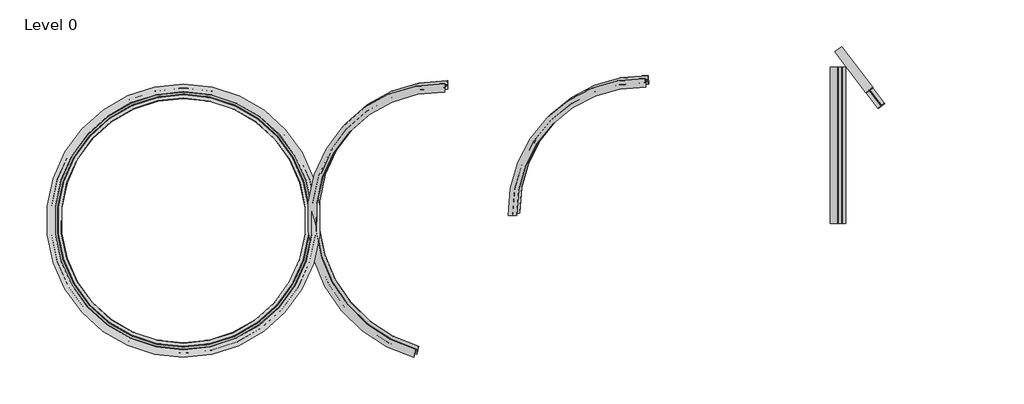
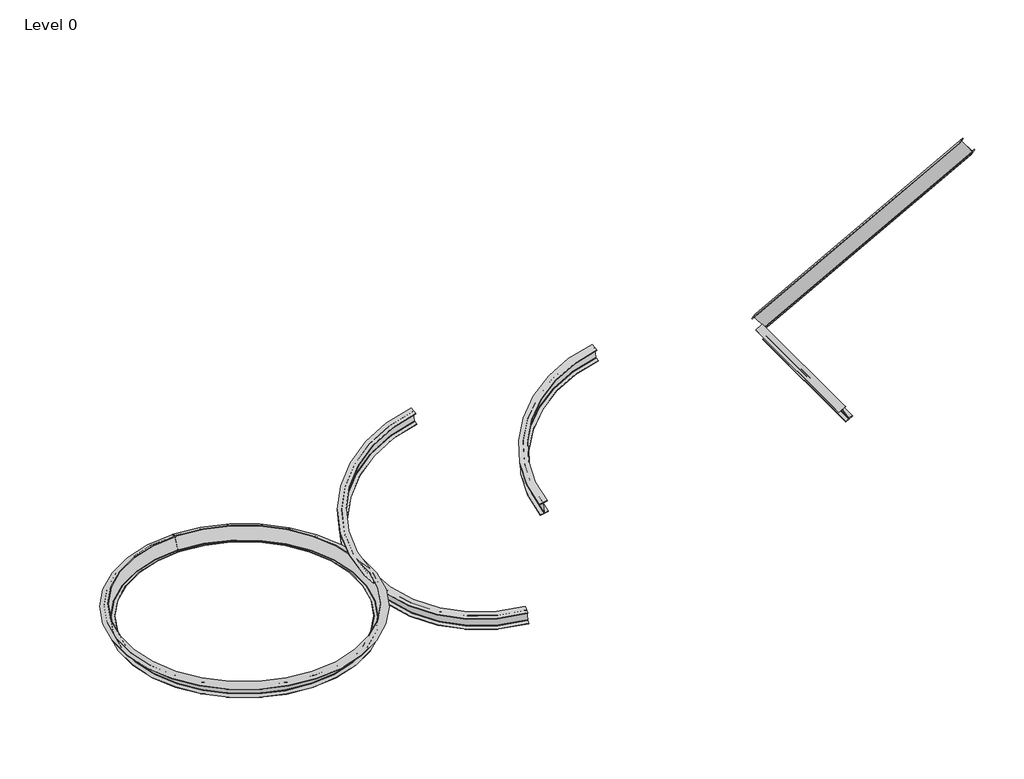
# One storey: 5 beams.
"""IFC4 building model written with IfcOpenShell, lengths in millimetres."""

import ifcopenshell
import ifcopenshell.guid

model = None  # the IFC model being written
_history = None  # IfcOwnerHistory: only IFC2X3 demands one
_inside = {}  # id of a spatial element -> (the spatial element, [elements in it])
_under = {}  # id of a project, library or spatial element -> (it, [spatial elements below it])
_declared = {}  # id of a project -> (the project, [libraries it declares])
_typed = {}  # id of a type object -> (the type object, [elements of that type])
_made_of = {}  # id of a material, layer set ... -> (it, [elements and type objects made of it])


def new_model(schema):
    """Start an empty IFC model of exactly this schema.

    Asked for "IFC4X3", IfcOpenShell would pick the latest addendum, in which some entities
    have other attributes; the version numbers below select the first issue.
    IFC2X3 requires an IfcOwnerHistory on every rooted entity: one is made here for all.
    """
    global model, _history
    if schema == "IFC4X3":
        model = ifcopenshell.file(schema_version=(4, 3, 0, 0))
    else:
        model = ifcopenshell.file(schema=schema)
    _inside.clear()
    _under.clear()
    _declared.clear()
    _typed.clear()
    _made_of.clear()
    _history = None
    if model.schema == "IFC2X3":
        org = make("IfcOrganization", Name="unknown")
        user = make(
            "IfcPersonAndOrganization",
            ThePerson=make("IfcPerson", FamilyName="unknown"),
            TheOrganization=org,
        )
        app = make(
            "IfcApplication",
            ApplicationDeveloper=org,
            Version="unknown",
            ApplicationFullName="unknown",
            ApplicationIdentifier="unknown",
        )
        _history = make(
            "IfcOwnerHistory",
            OwningUser=user,
            OwningApplication=app,
            ChangeAction="ADDED",
            CreationDate=0,
        )
    return model


def make(cls, **values):
    """One entity of the class cls with the attributes given. An attribute that is None is left unset."""
    return model.create_entity(
        cls, **{name: value for name, value in values.items() if value is not None}
    )


def rooted(cls, **values):
    """An entity with a GlobalId (a new one), such as an element, a storey or a relation."""
    return make(cls, GlobalId=ifcopenshell.guid.new(), OwnerHistory=_history, **values)


def si_unit(unit_type, name, prefix=None):
    """IfcSIUnit, for example si_unit("LENGTHUNIT", "METRE", prefix="MILLI")."""
    return make("IfcSIUnit", UnitType=unit_type, Prefix=prefix, Name=name)


def assignment(units):
    """IfcUnitAssignment: the units of a project."""
    return None if units is None else make("IfcUnitAssignment", Units=units)


def point(xyz):
    """IfcCartesianPoint."""
    return None if xyz is None else make("IfcCartesianPoint", Coordinates=xyz)


def direction(xyz):
    """IfcDirection."""
    return None if xyz is None else make("IfcDirection", DirectionRatios=xyz)


def frame(location, z_axis=None, x_axis=None):
    """IfcAxis2Placement3D, a coordinate frame: its origin and axes. An axis left out is left unset."""
    return make(
        "IfcAxis2Placement3D",
        Location=point(location),
        Axis=direction(z_axis),
        RefDirection=direction(x_axis),
    )


def frame_2d(location, x_axis=None):
    """IfcAxis2Placement2D, a coordinate frame in the plane: its origin and x axis."""
    return make(
        "IfcAxis2Placement2D", Location=point(location), RefDirection=direction(x_axis)
    )


def origin():
    """The frame at (0, 0, 0) with its axes left unset."""
    return frame((0.0, 0.0, 0.0))


def place(relative_to, where):
    """IfcLocalPlacement: puts the frame where relative to a parent placement (None: the world)."""
    return make(
        "IfcLocalPlacement", PlacementRelTo=relative_to, RelativePlacement=where
    )


def context(
    kind, dimensions, precision=None, world=None, true_north=None, identifier=None
):
    """IfcGeometricRepresentationContext, for example the 3D "Model" context."""
    return make(
        "IfcGeometricRepresentationContext",
        ContextIdentifier=identifier,
        ContextType=kind,
        CoordinateSpaceDimension=dimensions,
        Precision=precision,
        WorldCoordinateSystem=world,
        TrueNorth=true_north,
    )


def project(units=None, contexts=None):
    """IfcProject with its units and contexts."""
    return rooted(
        "IfcProject",
        Name="project",
        RepresentationContexts=contexts,
        UnitsInContext=assignment(units),
    )


def spatial(cls, under=None, at=None, **own):
    """A site, building, storey or space (cls), placed at a placement, below another one or the project."""
    s = rooted(cls, ObjectPlacement=at, **own)
    if under is not None:
        _under.setdefault(under.id(), (under, []))[1].append(s)
    return s


def polyline(points):
    """IfcPolyline through the points."""
    return make("IfcPolyline", Points=[point(p) for p in points])


def circle_curve(where, radius):
    """IfcCircle in the frame where."""
    return make("IfcCircle", Position=where, Radius=radius)


def ellipse_curve(where, semi_axis1, semi_axis2):
    """IfcEllipse in the frame where."""
    return make(
        "IfcEllipse", Position=where, SemiAxis1=semi_axis1, SemiAxis2=semi_axis2
    )


def trimmed(basis, trim1, trim2, sense, master):
    """IfcTrimmedCurve: the piece of a basis curve between two trims."""
    return make(
        "IfcTrimmedCurve",
        BasisCurve=basis,
        Trim1=trim1,
        Trim2=trim2,
        SenseAgreement=sense,
        MasterRepresentation=master,
    )


def segment(curve, same_sense, transition):
    """IfcCompositeCurveSegment."""
    return make(
        "IfcCompositeCurveSegment",
        Transition=transition,
        SameSense=same_sense,
        ParentCurve=curve,
    )


def composite_curve(segments, self_intersect=None):
    """IfcCompositeCurve: segments joined end to end."""
    return make("IfcCompositeCurve", Segments=segments, SelfIntersect=self_intersect)


def outline(outer, holes=None, kind="AREA"):
    """IfcArbitraryClosedProfileDef: a profile drawn as a closed curve; with holes, ...WithVoids."""
    if holes is None:
        return make("IfcArbitraryClosedProfileDef", ProfileType=kind, OuterCurve=outer)
    return make(
        "IfcArbitraryProfileDefWithVoids",
        ProfileType=kind,
        OuterCurve=outer,
        InnerCurves=holes,
    )


def extrude(swept, where, along, depth):
    """IfcExtrudedAreaSolid: the profile swept, set in the frame where, extruded along a direction by depth."""
    return make(
        "IfcExtrudedAreaSolid",
        SweptArea=swept,
        Position=where,
        ExtrudedDirection=direction(along),
        Depth=depth,
    )


def shape(context_of_items, identifier, shape_type, items):
    """IfcShapeRepresentation: the items that make up one representation, for example the "Body"."""
    return make(
        "IfcShapeRepresentation",
        ContextOfItems=context_of_items,
        RepresentationIdentifier=identifier,
        RepresentationType=shape_type,
        Items=items,
    )


def source(mapping_origin, context_of_items, identifier, shape_type, items):
    """IfcRepresentationMap: a shape defined once, which mapped items show again and again."""
    return make(
        "IfcRepresentationMap",
        MappingOrigin=mapping_origin,
        MappedRepresentation=shape(context_of_items, identifier, shape_type, items),
    )


def transform(
    local_origin,
    x_axis=None,
    y_axis=None,
    z_axis=None,
    scale=None,
    scale2=None,
    scale3=None,
    uniform=True,
):
    """IfcCartesianTransformationOperator3D, or its non-uniform kind. x_axis, y_axis, z_axis: its Axis1, 2, 3."""
    if uniform:
        return make(
            "IfcCartesianTransformationOperator3D",
            Axis1=direction(x_axis),
            Axis2=direction(y_axis),
            LocalOrigin=point(local_origin),
            Scale=scale,
            Axis3=direction(z_axis),
        )
    return make(
        "IfcCartesianTransformationOperator3DnonUniform",
        Axis1=direction(x_axis),
        Axis2=direction(y_axis),
        LocalOrigin=point(local_origin),
        Scale=scale,
        Axis3=direction(z_axis),
        Scale2=scale2,
        Scale3=scale3,
    )


def mapped(mapping_source, mapping_target):
    """IfcMappedItem: shows the shape of a source again, moved by a transform."""
    return make(
        "IfcMappedItem", MappingSource=mapping_source, MappingTarget=mapping_target
    )


def made_of(thing, what):
    """Note that an element or type object is made of a material, layer set ...; save() writes the relation."""
    if what is not None:
        _made_of.setdefault(what.id(), (what, []))[1].append(thing)
    return thing


def element(
    cls,
    number,
    at=None,
    inside=None,
    cuts=None,
    type_object=None,
    material=None,
    context=None,
    identifier="Body",
    shape_type=None,
    held_by="IfcProductDefinitionShape",
    body=None,
    shapes=None,
    **own,
):
    """One element of the class cls, such as IfcWall. Its Tag is "e" and its number.

    at: its placement. inside: the storey or other place that contains it. cuts: it is an
    opening in that element (IfcRelVoidsElement). A single representation is given by context,
    identifier, shape_type and body (its items); several are given by shapes. held_by: the class
    of the entity that holds the representations. save() writes the other relations.
    """
    e = rooted(cls, Tag="e%d" % number, ObjectPlacement=at, **own)
    if body is not None:
        shapes = [shape(context, identifier, shape_type, body)]
    if shapes is not None:
        e.Representation = make(held_by, Representations=shapes)
    if inside is not None:
        _inside.setdefault(inside.id(), (inside, []))[1].append(e)
    if cuts is not None:
        rooted(
            "IfcRelVoidsElement", RelatingBuildingElement=cuts, RelatedOpeningElement=e
        )
    if type_object is not None:
        _typed.setdefault(type_object.id(), (type_object, []))[1].append(e)
    return made_of(e, material)


def aggregate(whole, parts):
    """IfcRelAggregates: a whole, such as a stair, and the parts it consists of."""
    return rooted("IfcRelAggregates", RelatingObject=whole, RelatedObjects=parts)


def save(model, path):
    """Write the relations noted so far, then the file.

    IfcRelAggregates (storeys below a building ...), IfcRelContainedInSpatialStructure (elements
    in a storey), IfcRelDefinesByType, IfcRelAssociatesMaterial and IfcRelDeclares: one each for
    every whole, place, type object, material and project.
    """
    for whole, parts in _under.values():
        aggregate(whole, parts)
    for where, things in _inside.values():
        rooted(
            "IfcRelContainedInSpatialStructure",
            RelatedElements=things,
            RelatingStructure=where,
        )
    for kind, things in _typed.values():
        rooted("IfcRelDefinesByType", RelatedObjects=things, RelatingType=kind)
    for what, things in _made_of.values():
        rooted("IfcRelAssociatesMaterial", RelatedObjects=things, RelatingMaterial=what)
    for by, libraries in _declared.values():
        rooted("IfcRelDeclares", RelatingContext=by, RelatedDefinitions=libraries)
    model.write(path)


def plane_surface(at):
    """IfcPlane: the flat surface through the origin of the frame at, square to its z axis."""
    return make("IfcPlane", Position=at)


def cylinder_surface(at, radius):
    """IfcCylindricalSurface: all points at the distance radius from the z axis of the frame at."""
    return make("IfcCylindricalSurface", Position=at, Radius=radius)


def revolved_surface(curve, axis_point, axis_direction):
    """IfcSurfaceOfRevolution: the curve turned about the line through axis_point along axis_direction."""
    return make(
        "IfcSurfaceOfRevolution",
        SweptCurve=make("IfcArbitraryOpenProfileDef", ProfileType="CURVE", Curve=curve),
        AxisPosition=make("IfcAxis1Placement", Location=point(axis_point), Axis=direction(axis_direction)),
    )


def advanced_brep(points, edges, surfaces, faces):
    """IfcAdvancedBrep: a solid bounded by faces that lie on surfaces and meet in shared edges.

    An edge is (start, end): straight between two places in points (the first is 0);
    or (start, end, curve); or (start, end, curve, False) where it runs against its curve.
    A face is (place in surfaces, loops), or (place, loops, False) where it looks against
    its surface's normal. A loop lists edges by number (the first is 1), with a minus sign
    where the edge is run from its end to its start. The first loop is the outer one.
    """
    corners = [point(p) for p in points]
    vertices = [make("IfcVertexPoint", VertexGeometry=c) for c in corners]
    made = []
    for start, end, *more in edges:
        made.append(
            make(
                "IfcEdgeCurve",
                EdgeStart=vertices[start],
                EdgeEnd=vertices[end],
                EdgeGeometry=more[0] if more else make("IfcPolyline", Points=[corners[start], corners[end]]),
                SameSense=more[1] if len(more) > 1 else True,
            )
        )
    hull = []
    for where, loops, *sense in faces:
        bounds = []
        for j, loop in enumerate(loops):
            ring = [make("IfcOrientedEdge", EdgeElement=made[abs(k) - 1], Orientation=k > 0) for k in loop]
            bounds.append(
                make(
                    "IfcFaceOuterBound" if j == 0 else "IfcFaceBound",
                    Bound=make("IfcEdgeLoop", EdgeList=ring),
                    Orientation=True,
                )
            )
        hull.append(make("IfcAdvancedFace", Bounds=bounds, FaceSurface=surfaces[where], SameSense=sense[0] if sense else True))
    return make("IfcAdvancedBrep", Outer=make("IfcClosedShell", CfsFaces=hull))


def ub_universal_beams_ub305x165x40_8b2c45c1(model_context):
    return source(origin(), model_context, "Body", "SweptSolid", [
        extrude(outline(composite_curve([segment(polyline([(82.5, -141.5), (82.5, -151.7), (-82.5, -151.7), (-82.5, -141.5), (-11.9, -141.5)]), True, "CONTINUOUS"), segment(trimmed(circle_curve(frame_2d((-11.9, -132.6)), 8.9), [point((-11.9, -141.5))], [point((-3.0, -132.6))], True, "CARTESIAN"), True, "CONTINUOUS"), segment(polyline([(-3.0, -132.6), (-3.0, 132.6)]), True, "CONTINUOUS"), segment(trimmed(circle_curve(frame_2d((-11.9, 132.6)), 8.9), [point((-3.0, 132.6))], [point((-11.9, 141.5))], True, "CARTESIAN"), True, "CONTINUOUS"), segment(polyline([(-11.9, 141.5), (-82.5, 141.5), (-82.5, 151.7), (82.5, 151.7), (82.5, 141.5), (11.9, 141.5)]), True, "CONTINUOUS"), segment(trimmed(circle_curve(frame_2d((11.9, 132.6)), 8.9), [point((11.9, 141.5))], [point((3.0, 132.6))], True, "CARTESIAN"), True, "CONTINUOUS"), segment(polyline([(3.0, 132.6), (3.0, -132.6)]), True, "CONTINUOUS"), segment(trimmed(circle_curve(frame_2d((11.9, -132.6)), 8.9), [point((3.0, -132.6))], [point((11.9, -141.5))], True, "CARTESIAN"), True, "CONTINUOUS"), segment(polyline([(11.9, -141.5), (82.5, -141.5)]), True, "CONTINUOUS")], self_intersect=False)), frame((-1500.0, 0.0, 0.0), z_axis=(1.0, 0.0, 0.0), x_axis=(0.0, 1.0, 0.0)), (0.0, 0.0, 1.0), 3000.0),
    ])


def ub_universal_beams_ub305x165x40_614cc3fe(model_context):
    return source(origin(), model_context, "Body", "SweptSolid", [
        extrude(outline(composite_curve([segment(polyline([(82.5, -141.5), (82.5, -151.7), (-82.5, -151.7), (-82.5, -141.5), (-11.9, -141.5)]), True, "CONTINUOUS"), segment(trimmed(circle_curve(frame_2d((-11.9, -132.6)), 8.9), [point((-11.9, -141.5))], [point((-3.0, -132.6))], True, "CARTESIAN"), True, "CONTINUOUS"), segment(polyline([(-3.0, -132.6), (-3.0, 132.6)]), True, "CONTINUOUS"), segment(trimmed(circle_curve(frame_2d((-11.9, 132.6)), 8.9), [point((-3.0, 132.6))], [point((-11.9, 141.5))], True, "CARTESIAN"), True, "CONTINUOUS"), segment(polyline([(-11.9, 141.5), (-82.5, 141.5), (-82.5, 151.7), (82.5, 151.7), (82.5, 141.5), (11.9, 141.5)]), True, "CONTINUOUS"), segment(trimmed(circle_curve(frame_2d((11.9, 132.6)), 8.9), [point((11.9, 141.5))], [point((3.0, 132.6))], True, "CARTESIAN"), True, "CONTINUOUS"), segment(polyline([(3.0, 132.6), (3.0, -132.6)]), True, "CONTINUOUS"), segment(trimmed(circle_curve(frame_2d((11.9, -132.6)), 8.9), [point((3.0, -132.6))], [point((11.9, -141.5))], True, "CARTESIAN"), True, "CONTINUOUS"), segment(polyline([(11.9, -141.5), (82.5, -141.5)]), True, "CONTINUOUS")], self_intersect=False)), frame((-3226.45, 0.0, 0.0), z_axis=(1.0, 0.0, 0.0), x_axis=(0.0, 1.0, 0.0)), (0.0, 0.0, 1.0), 6452.9),
    ])


def ub_universal_beams_ub305x165x40_b211cafa(model_context):
    return source(origin(), model_context, "Body", "AdvancedBrep", [
        advanced_brep(
        [(-9.2813175, 14.9526552, -163.1085585), (-9.0434318, -49.0322323, -133.2717092), (-9.0274272, -53.3370394, -121.4442673), (-9.444114, 58.7405491, 118.9085578), (-9.4880863, 70.5679092, 123.2133946), (-9.725972, 134.5527967, 93.3765453), (-9.7419984, 138.8634732, 102.6208847), (-9.1860332, -10.6762782, 172.3528979), (-9.1700068, -14.9869547, 163.1085585), (-9.4078925, 48.9979329, 133.2717092), (-9.4238971, 53.3027399, 121.4442673), (-9.0072103, -58.7748485, -118.9085578), (-8.9632381, -70.6022086, -123.2133946), (-8.7253523, -134.5870962, -93.3765453), (-8.7093259, -138.8977726, -102.6208847), (-9.2652911, 10.6419787, -172.3528979), (0.0, 14.9699084, -163.1085585), (0.0, 10.6592021, -172.3528979), (0.0, -138.8815827, -102.6208847), (0.0, -134.5708765, -93.3765453), (0.0, -70.5855467, -123.2133946), (0.0, -58.7581049, -118.9085578), (0.0, 53.3202581, 121.4442673), (0.0, 49.0154214, 133.2717092), (0.0, -14.9699084, 163.1085585), (0.0, -10.6592021, 172.3528979), (0.0, 138.8815827, 102.6208847), (0.0, 134.5708765, 93.3765453), (0.0, 70.5855467, 123.2133946), (0.0, 58.7581049, 118.9085578), (0.0, -53.3202581, -121.4442673), (0.0, -49.0154214, -133.2717092)],
        [
            (0, 1),
            (1, 2, circle_curve(frame((-9.0574157, -45.2709558, -125.2055699), z_axis=(-0.9999930888962334, -0.0037178165326446095, 0.0), x_axis=(0.0033694860743094072, -0.9063015234494892, 0.4226182617406991)), 8.9)),
            (2, 3),
            (3, 4, circle_curve(frame((-9.4741024, 66.8066326, 115.1472552), z_axis=(-0.9999930888962334, -0.0037178165326453875, 0.0), x_axis=(0.003369486074310112, -0.9063015234494892, 0.42261826174069916)), 8.9)),
            (4, 5),
            (5, 6),
            (6, 7),
            (7, 8),
            (8, 9),
            (9, 10, circle_curve(frame((-9.3939087, 45.2366564, 125.2055699), z_axis=(-0.9999930888962334, -0.0037178165326453875, 0.0), x_axis=(0.003369486074310112, -0.9063015234494892, 0.42261826174069916)), 8.9)),
            (10, 11),
            (11, 12, circle_curve(frame((-8.9772219, -66.8409321, -115.1472552), z_axis=(-0.9999930888962334, -0.0037178165326446095, 0.0), x_axis=(0.0033694860743094072, -0.9063015234494892, 0.4226182617406991)), 8.9)),
            (12, 13),
            (13, 14),
            (14, 15),
            (15, 0),
            (16, 17),
            (17, 18),
            (18, 19),
            (19, 20),
            (20, 21, circle_curve(frame((0.0, -66.8242442, -115.1472552), z_axis=(1.0000000000000002, 0.0, 0.0), x_axis=(0.0, -0.9063077870366502, 0.4226182617406991)), 8.9)),
            (21, 22),
            (22, 23, circle_curve(frame((0.0, 45.2541188, 125.2055699), z_axis=(1.0000000000000002, 0.0, 0.0), x_axis=(0.0, -0.9063077870366502, 0.42261826174069916)), 8.9)),
            (23, 24),
            (24, 25),
            (25, 26),
            (26, 27),
            (27, 28),
            (28, 29, circle_curve(frame((0.0, 66.8242442, 115.1472552), z_axis=(1.0000000000000002, 0.0, 0.0), x_axis=(0.0, -0.9063077870366502, 0.42261826174069916)), 8.9)),
            (29, 30),
            (30, 31, circle_curve(frame((0.0, -45.2541188, -125.2055699), z_axis=(1.0000000000000002, 0.0, 0.0), x_axis=(0.0, -0.9063077870366502, 0.4226182617406991)), 8.9)),
            (31, 16),
            (0, 16, circle_curve(frame((0.0, -2481.473222, -163.1085585), z_axis=(0.0, 0.0, 1.0), x_axis=(-0.9999930888962332, -0.0037178165326318038, 0.0)), 2496.4431304)),
            (31, 1, circle_curve(frame((0.0, -2481.473222, -133.2717092), z_axis=(0.0, 0.0, -1.0), x_axis=(-0.9999930888962332, -0.0037178165326318038, 0.0)), 2432.4578006)),
            (30, 2, circle_curve(frame((0.0, -2481.473222, -121.4442673), z_axis=(0.0, 0.0, -1.0), x_axis=(-0.9999930888962332, -0.0037178165326318038, 0.0)), 2428.1529638)),
            (29, 3, circle_curve(frame((0.0, -2481.473222, 118.9085578), z_axis=(0.0, 0.0, -1.0), x_axis=(-0.9999930888962332, -0.0037178165326318038, 0.0)), 2540.2313268)),
            (28, 4, circle_curve(frame((0.0, -2481.473222, 123.2133946), z_axis=(0.0, 0.0, -1.0), x_axis=(-0.9999930888962332, -0.0037178165326318038, 0.0)), 2552.0587687)),
            (27, 5, circle_curve(frame((0.0, -2481.473222, 93.3765453), z_axis=(0.0, 0.0, -1.0), x_axis=(-0.9999930888962332, -0.0037178165326318038, 0.0)), 2616.0440984)),
            (26, 6, circle_curve(frame((0.0, -2481.473222, 102.6208847), z_axis=(0.0, 0.0, -1.0), x_axis=(-0.9999930888962332, -0.0037178165326318038, 0.0)), 2620.3548047)),
            (25, 7, circle_curve(frame((0.0, -2481.473222, 172.3528979), z_axis=(0.0, 0.0, -1.0), x_axis=(-0.9999930888962332, -0.0037178165326318038, 0.0)), 2470.8140198)),
            (24, 8, circle_curve(frame((0.0, -2481.473222, 163.1085585), z_axis=(0.0, 0.0, -1.0), x_axis=(-0.9999930888962332, -0.0037178165326318038, 0.0)), 2466.5033136)),
            (23, 9, circle_curve(frame((0.0, -2481.473222, 133.2717092), z_axis=(0.0, 0.0, -1.0), x_axis=(-0.9999930888962332, -0.0037178165326318038, 0.0)), 2530.4886433)),
            (22, 10, circle_curve(frame((0.0, -2481.473222, 121.4442673), z_axis=(0.0, 0.0, -1.0), x_axis=(-0.9999930888962332, -0.0037178165326318038, 0.0)), 2534.7934801)),
            (21, 11, circle_curve(frame((0.0, -2481.473222, -118.9085578), z_axis=(0.0, 0.0, -1.0), x_axis=(-0.9999930888962332, -0.0037178165326318038, 0.0)), 2422.7151171)),
            (20, 12, circle_curve(frame((0.0, -2481.473222, -123.2133946), z_axis=(0.0, 0.0, -1.0), x_axis=(-0.9999930888962332, -0.0037178165326318038, 0.0)), 2410.8876753)),
            (19, 13, circle_curve(frame((0.0, -2481.473222, -93.3765453), z_axis=(0.0, 0.0, -1.0), x_axis=(-0.9999930888962332, -0.0037178165326318038, 0.0)), 2346.9023455)),
            (18, 14, circle_curve(frame((0.0, -2481.473222, -102.6208847), z_axis=(0.0, 0.0, -1.0), x_axis=(-0.9999930888962332, -0.0037178165326318038, 0.0)), 2342.5916392)),
            (17, 15, circle_curve(frame((0.0, -2481.473222, -172.3528979), z_axis=(0.0, 0.0, -1.0), x_axis=(-0.9999930888962332, -0.0037178165326318038, 0.0)), 2492.1324241)),
        ],
        [
            plane_surface(frame((-9.2256622, -0.0171497, 0.0), z_axis=(0.9999930888962332, 0.0037178165326321104, 0.0), x_axis=(-0.0015712171604918153, 0.42261534098203835, 0.9063077870366502))),
            plane_surface(frame((0.0, 0.0, 0.0), z_axis=(-1.0, 0.0, 0.0), x_axis=(0.0, 0.422618261740699, 0.9063077870366502))),
            revolved_surface(polyline([(-2432.4409896, -2490.5166538, -133.2717092), (-2496.4258772, -2490.7545395, -163.1085585)]), (0.0, -2481.473222, 0.0), (0.0, 0.0, -1.0)),
            revolved_surface(trimmed(ellipse_curve(frame((-2436.2022662, -2490.5306376, -125.2055699), z_axis=(-0.0037178165326371983, 0.9999930888962334, 0.0), x_axis=(0.9063015234494892, 0.00336948607430269, 0.4226182617406992)), 8.9, 8.9), [point((-2428.1361826, -2490.5006492, -121.4442673))], [point((-2432.4409896, -2490.5166538, -133.2717092))], True, "CARTESIAN"), (0.0, -2481.473222, 0.0), (0.0, 0.0, -1.0)),
            revolved_surface(polyline([(-2540.213771, -2490.917336, 118.9085578), (-2428.1361826, -2490.5006492, -121.4442673)]), (0.0, -2481.473222, 0.0), (0.0, 0.0, -1.0)),
            revolved_surface(trimmed(ellipse_curve(frame((-2548.2798546, -2490.9473244, 115.1472552), z_axis=(-0.003717816532637976, 0.9999930888962334, 0.0), x_axis=(0.9063015234494892, 0.0033694860743033947, 0.4226182617406993)), 8.9, 8.9), [point((-2552.0411311, -2490.9613082, 123.2133946))], [point((-2540.213771, -2490.917336, 118.9085578))], True, "CARTESIAN"), (0.0, -2481.473222, 0.0), (0.0, 0.0, -1.0)),
            revolved_surface(polyline([(-2616.0260187, -2491.199194, 93.3765453), (-2552.0411311, -2490.9613082, 123.2133946)]), (0.0, -2481.473222, 0.0), (0.0, 0.0, -1.0)),
            revolved_surface(polyline([(-2620.3366952, -2491.2152204, 102.6208847), (-2616.0260187, -2491.199194, 93.3765453)]), (0.0, -2481.473222, 0.0), (0.0, 0.0, -1.0)),
            revolved_surface(polyline([(-2470.7969438, -2490.6592552, 172.3528979), (-2620.3366952, -2491.2152204, 102.6208847)]), (0.0, -2481.473222, 0.0), (0.0, 0.0, -1.0)),
            revolved_surface(polyline([(-2466.4862673, -2490.6432288, 163.1085585), (-2470.7969438, -2490.6592552, 172.3528979)]), (0.0, -2481.473222, 0.0), (0.0, 0.0, -1.0)),
            revolved_surface(polyline([(-2530.4711549, -2490.8811145, 133.2717092), (-2466.4862673, -2490.6432288, 163.1085585)]), (0.0, -2481.473222, 0.0), (0.0, 0.0, -1.0)),
            revolved_surface(trimmed(ellipse_curve(frame((-2526.7098783, -2490.8671306, 125.2055699), z_axis=(-0.003717816532637976, 0.9999930888962334, 0.0), x_axis=(0.9063015234494892, 0.0033694860743033947, 0.4226182617406993)), 8.9, 8.9), [point((-2534.7759619, -2490.8971191, 121.4442673))], [point((-2530.4711549, -2490.8811145, 133.2717092))], True, "CARTESIAN"), (0.0, -2481.473222, 0.0), (0.0, 0.0, -1.0)),
            revolved_surface(polyline([(-2422.6983735, -2490.4804323, -118.9085578), (-2534.7759619, -2490.8971191, 121.4442673)]), (0.0, -2481.473222, 0.0), (0.0, 0.0, -1.0)),
            revolved_surface(trimmed(ellipse_curve(frame((-2414.6322899, -2490.4504439, -115.1472552), z_axis=(-0.0037178165326371983, 0.9999930888962334, 0.0), x_axis=(0.9063015234494892, 0.00336948607430269, 0.4226182617406992)), 8.9, 8.9), [point((-2410.8710134, -2490.43646, -123.2133946))], [point((-2422.6983735, -2490.4804323, -118.9085578))], True, "CARTESIAN"), (0.0, -2481.473222, 0.0), (0.0, 0.0, -1.0)),
            revolved_surface(polyline([(-2346.8861258, -2490.1985743, -93.3765453), (-2410.8710134, -2490.43646, -123.2133946)]), (0.0, -2481.473222, 0.0), (0.0, 0.0, -1.0)),
            revolved_surface(polyline([(-2342.5754493, -2490.1825479, -102.6208847), (-2346.8861258, -2490.1985743, -93.3765453)]), (0.0, -2481.473222, 0.0), (0.0, 0.0, -1.0)),
            revolved_surface(polyline([(-2492.1152007, -2490.7385131, -172.3528979), (-2342.5754493, -2490.1825479, -102.6208847)]), (0.0, -2481.473222, 0.0), (0.0, 0.0, -1.0)),
            revolved_surface(polyline([(-2496.4258772, -2490.7545395, -163.1085585), (-2492.1152007, -2490.7385131, -172.3528979)]), (0.0, -2481.473222, 0.0), (0.0, 0.0, -1.0)),
        ],
        [
            (0, [[1, 2, 3, 4, 5, 6, 7, 8, 9, 10, 11, 12, 13, 14, 15, 16]]),
            (1, [[17, 18, 19, 20, 21, 22, 23, 24, 25, 26, 27, 28, 29, 30, 31, 32]]),
            (2, [[-1, 33, -32, 34]]),
            (3, [[-2, -34, -31, 35]]),
            (4, [[-3, -35, -30, 36]]),
            (5, [[-4, -36, -29, 37]]),
            (6, [[-5, -37, -28, 38]]),
            (7, [[-6, -38, -27, 39]]),
            (8, [[-7, -39, -26, 40]]),
            (9, [[-8, -40, -25, 41]]),
            (10, [[-9, -41, -24, 42]]),
            (11, [[-10, -42, -23, 43]]),
            (12, [[-11, -43, -22, 44]]),
            (13, [[-12, -44, -21, 45]]),
            (14, [[-13, -45, -20, 46]]),
            (15, [[-14, -46, -19, 47]]),
            (16, [[-15, -47, -18, 48]]),
            (17, [[-16, -48, -17, -33]]),
        ],
    ),
    ])


def ub_universal_beams_ub305x165x40_4e4f8f72(model_context):
    return source(origin(), model_context, "Body", "AdvancedBrep", [
        advanced_brep(
        [(2724.4689627, -2641.9689627, -141.5), (2653.8689627, -2641.9689627, -141.5), (2644.9689627, -2641.9689627, -132.6), (2644.9689627, -2641.9689627, 132.6), (2653.8689627, -2641.9689627, 141.5), (2724.4689627, -2641.9689627, 141.5), (2724.4689627, -2641.9689627, 151.7), (2559.4689627, -2641.9689627, 151.7), (2559.4689627, -2641.9689627, 141.5), (2630.0689627, -2641.9689627, 141.5), (2638.9689627, -2641.9689627, 132.6), (2638.9689627, -2641.9689627, -132.6), (2630.0689627, -2641.9689627, -141.5), (2559.4689627, -2641.9689627, -141.5), (2559.4689627, -2641.9689627, -151.7), (2724.4689627, -2641.9689627, -151.7), (-2633.0924312, -1942.2866222, -141.5), (-2633.0924312, -1942.2866222, -151.7), (-2473.6264005, -1984.6609666, -151.7), (-2473.6264005, -1984.6609666, -141.5), (-2541.8585324, -1966.5298835, -141.5), (-2550.4600335, -1964.244237, -132.6), (-2550.4600335, -1964.244237, 132.6), (-2541.8585324, -1966.5298835, 141.5), (-2473.6264005, -1984.6609666, 141.5), (-2473.6264005, -1984.6609666, 151.7), (-2633.0924312, -1942.2866222, 151.7), (-2633.0924312, -1942.2866222, 141.5), (-2564.8602993, -1960.4177053, 141.5), (-2556.2587982, -1962.7033518, 132.6), (-2556.2587982, -1962.7033518, -132.6), (-2564.8602993, -1960.4177053, -141.5)],
        [
            (0, 1),
            (1, 2, circle_curve(frame((2653.8689627, -2641.9689627, -132.6), z_axis=(0.0, 1.0, 0.0), x_axis=(-1.0, 0.0, 0.0)), 8.9)),
            (2, 3),
            (3, 4, circle_curve(frame((2653.8689627, -2641.9689627, 132.6), z_axis=(0.0, 1.0, 0.0), x_axis=(-1.0, 0.0, 0.0)), 8.9)),
            (4, 5),
            (5, 6),
            (6, 7),
            (7, 8),
            (8, 9),
            (9, 10, circle_curve(frame((2630.0689627, -2641.9689627, 132.6), z_axis=(0.0, 1.0, 0.0), x_axis=(-1.0, 0.0, 0.0)), 8.9)),
            (10, 11),
            (11, 12, circle_curve(frame((2630.0689627, -2641.9689627, -132.6), z_axis=(0.0, 1.0, 0.0), x_axis=(-1.0, 0.0, 0.0)), 8.9)),
            (12, 13),
            (13, 14),
            (14, 15),
            (15, 0),
            (16, 17),
            (17, 18),
            (18, 19),
            (19, 20),
            (20, 21, circle_curve(frame((-2541.8585324, -1966.5298835, -132.6), z_axis=(0.2568142086103926, 0.9664607918875021, 0.0), x_axis=(0.9664607918875021, -0.2568142086103926, 0.0)), 8.9)),
            (21, 22),
            (22, 23, circle_curve(frame((-2541.8585324, -1966.5298835, 132.6), z_axis=(0.2568142086103926, 0.9664607918875021, 0.0), x_axis=(0.9664607918875021, -0.2568142086103926, 0.0)), 8.9)),
            (23, 24),
            (24, 25),
            (25, 26),
            (26, 27),
            (27, 28),
            (28, 29, circle_curve(frame((-2564.8602993, -1960.4177053, 132.6), z_axis=(0.2568142086103926, 0.9664607918875021, 0.0), x_axis=(0.9664607918875021, -0.2568142086103926, 0.0)), 8.9)),
            (29, 30),
            (30, 31, circle_curve(frame((-2564.8602993, -1960.4177053, -132.6), z_axis=(0.2568142086103926, 0.9664607918875021, 0.0), x_axis=(0.9664607918875021, -0.2568142086103926, 0.0)), 8.9)),
            (31, 16),
            (0, 16, circle_curve(frame((0.0, -2641.9689627, -141.5), z_axis=(0.0, 0.0, 1.0), x_axis=(0.0, 1.0, 0.0)), 2724.4689627)),
            (31, 1, circle_curve(frame((0.0, -2641.9689627, -141.5), z_axis=(0.0, 0.0, -1.0), x_axis=(0.0, 1.0, 0.0)), 2653.8689627)),
            (30, 2, circle_curve(frame((0.0, -2641.9689627, -132.6), z_axis=(0.0, 0.0, -1.0), x_axis=(0.0, 1.0, 0.0)), 2644.9689627)),
            (29, 3, circle_curve(frame((0.0, -2641.9689627, 132.6), z_axis=(0.0, 0.0, -1.0), x_axis=(0.0, 1.0, 0.0)), 2644.9689627)),
            (28, 4, circle_curve(frame((0.0, -2641.9689627, 141.5), z_axis=(0.0, 0.0, -1.0), x_axis=(0.0, 1.0, 0.0)), 2653.8689627)),
            (27, 5, circle_curve(frame((0.0, -2641.9689627, 141.5), z_axis=(0.0, 0.0, -1.0), x_axis=(0.0, 1.0, 0.0)), 2724.4689627)),
            (26, 6, circle_curve(frame((0.0, -2641.9689627, 151.7), z_axis=(0.0, 0.0, -1.0), x_axis=(0.0, 1.0, 0.0)), 2724.4689627)),
            (25, 7, circle_curve(frame((0.0, -2641.9689627, 151.7), z_axis=(0.0, 0.0, -1.0), x_axis=(0.0, 1.0, 0.0)), 2559.4689627)),
            (24, 8, circle_curve(frame((0.0, -2641.9689627, 141.5), z_axis=(0.0, 0.0, -1.0), x_axis=(0.0, 1.0, 0.0)), 2559.4689627)),
            (23, 9, circle_curve(frame((0.0, -2641.9689627, 141.5), z_axis=(0.0, 0.0, -1.0), x_axis=(0.0, 1.0, 0.0)), 2630.0689627)),
            (22, 10, circle_curve(frame((0.0, -2641.9689627, 132.6), z_axis=(0.0, 0.0, -1.0), x_axis=(0.0, 1.0, 0.0)), 2638.9689627)),
            (21, 11, circle_curve(frame((0.0, -2641.9689627, -132.6), z_axis=(0.0, 0.0, -1.0), x_axis=(0.0, 1.0, 0.0)), 2638.9689627)),
            (20, 12, circle_curve(frame((0.0, -2641.9689627, -141.5), z_axis=(0.0, 0.0, -1.0), x_axis=(0.0, 1.0, 0.0)), 2630.0689627)),
            (19, 13, circle_curve(frame((0.0, -2641.9689627, -141.5), z_axis=(0.0, 0.0, -1.0), x_axis=(0.0, 1.0, 0.0)), 2559.4689627)),
            (18, 14, circle_curve(frame((0.0, -2641.9689627, -151.7), z_axis=(0.0, 0.0, -1.0), x_axis=(0.0, 1.0, 0.0)), 2559.4689627)),
            (17, 15, circle_curve(frame((0.0, -2641.9689627, -151.7), z_axis=(0.0, 0.0, -1.0), x_axis=(0.0, 1.0, 0.0)), 2724.4689627)),
        ],
        [
            plane_surface(frame((2641.9689627, -2641.9689627, 0.0), z_axis=(0.0, -1.0, 0.0), x_axis=(0.0, 0.0, 1.0))),
            plane_surface(frame((-2553.3594159, -1963.4737944, 0.0), z_axis=(-0.25681420861039306, -0.9664607918875021, 0.0), x_axis=(0.0, 0.0, 1.0))),
            plane_surface(frame((0.0, -2641.9689627, -141.5), z_axis=(0.0, 0.0, 1.0), x_axis=(0.0, 1.0, 0.0))),
            revolved_surface(trimmed(ellipse_curve(frame((0.0, 11.9, -132.6), z_axis=(1.0, 0.0, 0.0), x_axis=(0.0, -1.0, 0.0)), 8.9, 8.9), [point((0.0, 3.0, -132.6))], [point((0.0, 11.9, -141.5))], True, "CARTESIAN"), (0.0, -2641.9689627, 0.0), (0.0, 0.0, -1.0)),
            cylinder_surface(frame((0.0, -2641.9689627, 0.0), z_axis=(0.0, 0.0, -1.0), x_axis=(0.0, 1.0, 0.0)), 2644.9689627),
            revolved_surface(trimmed(ellipse_curve(frame((0.0, 11.9, 132.6), z_axis=(1.0, 0.0, 0.0), x_axis=(0.0, -1.0, 0.0)), 8.9, 8.9), [point((0.0, 11.9, 141.5))], [point((0.0, 3.0, 132.6))], True, "CARTESIAN"), (0.0, -2641.9689627, 0.0), (0.0, 0.0, -1.0)),
            plane_surface(frame((0.0, -2641.9689627, 141.5), z_axis=(0.0, 0.0, -1.0), x_axis=(0.0, 1.0, 0.0))),
            cylinder_surface(frame((0.0, -2641.9689627, 0.0), z_axis=(0.0, 0.0, -1.0), x_axis=(0.0, 1.0, 0.0)), 2724.4689627),
            plane_surface(frame((0.0, -2641.9689627, 151.7), z_axis=(0.0, 0.0, 1.0), x_axis=(0.0, 1.0, 0.0))),
            revolved_surface(polyline([(0.0, -82.5, 141.5), (0.0, -82.5, 151.7)]), (0.0, -2641.9689627, 0.0), (0.0, 0.0, -1.0)),
            revolved_surface(trimmed(ellipse_curve(frame((0.0, -11.9, 132.6), z_axis=(1.0, 0.0, 0.0), x_axis=(0.0, -1.0, 0.0)), 8.9, 8.9), [point((0.0, -3.0, 132.6))], [point((0.0, -11.9, 141.5))], True, "CARTESIAN"), (0.0, -2641.9689627, 0.0), (0.0, 0.0, -1.0)),
            revolved_surface(polyline([(0.0, -3.0, -132.6), (0.0, -3.0, 132.6)]), (0.0, -2641.9689627, 0.0), (0.0, 0.0, -1.0)),
            revolved_surface(trimmed(ellipse_curve(frame((0.0, -11.9, -132.6), z_axis=(1.0, 0.0, 0.0), x_axis=(0.0, -1.0, 0.0)), 8.9, 8.9), [point((0.0, -11.9, -141.5))], [point((0.0, -3.0, -132.6))], True, "CARTESIAN"), (0.0, -2641.9689627, 0.0), (0.0, 0.0, -1.0)),
            revolved_surface(polyline([(0.0, -82.5, -151.7), (0.0, -82.5, -141.5)]), (0.0, -2641.9689627, 0.0), (0.0, 0.0, -1.0)),
            plane_surface(frame((0.0, -2641.9689627, -151.7), z_axis=(0.0, 0.0, -1.0), x_axis=(0.0, 1.0, 0.0))),
        ],
        [
            (0, [[1, 2, 3, 4, 5, 6, 7, 8, 9, 10, 11, 12, 13, 14, 15, 16]]),
            (1, [[17, 18, 19, 20, 21, 22, 23, 24, 25, 26, 27, 28, 29, 30, 31, 32]]),
            (2, [[-1, 33, -32, 34]]),
            (3, [[-2, -34, -31, 35]]),
            (4, [[-3, -35, -30, 36]]),
            (5, [[-4, -36, -29, 37]]),
            (6, [[-5, -37, -28, 38]]),
            (7, [[-6, -38, -27, 39]]),
            (8, [[-7, -39, -26, 40]]),
            (9, [[-8, -40, -25, 41]]),
            (6, [[-9, -41, -24, 42]]),
            (10, [[-10, -42, -23, 43]]),
            (11, [[-11, -43, -22, 44]]),
            (12, [[-12, -44, -21, 45]]),
            (2, [[-13, -45, -20, 46]]),
            (13, [[-14, -46, -19, 47]]),
            (14, [[-15, -47, -18, 48]]),
            (7, [[-16, -48, -17, -33]]),
        ],
    ),
    ])


def ub_universal_beams_ub305x165x40_a7bc032b(model_context):
    return source(origin(), model_context, "Body", "AdvancedBrep", [
        advanced_brep(
        [(2724.4689627, -2641.9689627, -141.5), (2653.8689627, -2641.9689627, -141.5), (2644.9689627, -2641.9689627, -132.6), (2644.9689627, -2641.9689627, 132.6), (2653.8689627, -2641.9689627, 141.5), (2724.4689627, -2641.9689627, 141.5), (2724.4689627, -2641.9689627, 151.7), (2559.4689627, -2641.9689627, 151.7), (2559.4689627, -2641.9689627, 141.5), (2630.0689627, -2641.9689627, 141.5), (2638.9689627, -2641.9689627, 132.6), (2638.9689627, -2641.9689627, -132.6), (2630.0689627, -2641.9689627, -141.5), (2559.4689627, -2641.9689627, -141.5), (2559.4689627, -2641.9689627, -151.7), (2724.4689627, -2641.9689627, -151.7), (0.0, 82.5, -141.5), (0.0, 82.5, -151.7), (0.0, -82.5, -151.7), (0.0, -82.5, -141.5), (0.0, -11.9, -141.5), (0.0, -3.0, -132.6), (0.0, -3.0, 132.6), (0.0, -11.9, 141.5), (0.0, -82.5, 141.5), (0.0, -82.5, 151.7), (0.0, 82.5, 151.7), (0.0, 82.5, 141.5), (0.0, 11.9, 141.5), (0.0, 3.0, 132.6), (0.0, 3.0, -132.6), (0.0, 11.9, -141.5)],
        [
            (0, 1),
            (1, 2, circle_curve(frame((2653.8689627, -2641.9689627, -132.6), z_axis=(0.0, 1.0, 0.0), x_axis=(-1.0, 0.0, 0.0)), 8.9)),
            (2, 3),
            (3, 4, circle_curve(frame((2653.8689627, -2641.9689627, 132.6), z_axis=(0.0, 1.0, 0.0), x_axis=(-1.0, 0.0, 0.0)), 8.9)),
            (4, 5),
            (5, 6),
            (6, 7),
            (7, 8),
            (8, 9),
            (9, 10, circle_curve(frame((2630.0689627, -2641.9689627, 132.6), z_axis=(0.0, 1.0, 0.0), x_axis=(-1.0, 0.0, 0.0)), 8.9)),
            (10, 11),
            (11, 12, circle_curve(frame((2630.0689627, -2641.9689627, -132.6), z_axis=(0.0, 1.0, 0.0), x_axis=(-1.0, 0.0, 0.0)), 8.9)),
            (12, 13),
            (13, 14),
            (14, 15),
            (15, 0),
            (16, 17),
            (17, 18),
            (18, 19),
            (19, 20),
            (20, 21, circle_curve(frame((0.0, -11.9, -132.6), z_axis=(1.0, 0.0, 0.0), x_axis=(0.0, -1.0, 0.0)), 8.9)),
            (21, 22),
            (22, 23, circle_curve(frame((0.0, -11.9, 132.6), z_axis=(1.0, 0.0, 0.0), x_axis=(0.0, -1.0, 0.0)), 8.9)),
            (23, 24),
            (24, 25),
            (25, 26),
            (26, 27),
            (27, 28),
            (28, 29, circle_curve(frame((0.0, 11.9, 132.6), z_axis=(1.0, 0.0, 0.0), x_axis=(0.0, -1.0, 0.0)), 8.9)),
            (29, 30),
            (30, 31, circle_curve(frame((0.0, 11.9, -132.6), z_axis=(1.0, 0.0, 0.0), x_axis=(0.0, -1.0, 0.0)), 8.9)),
            (31, 16),
            (0, 16, circle_curve(frame((0.0, -2641.9689627, -141.5), z_axis=(0.0, 0.0, 1.0), x_axis=(0.0, 1.0, 0.0)), 2724.4689627)),
            (31, 1, circle_curve(frame((0.0, -2641.9689627, -141.5), z_axis=(0.0, 0.0, -1.0), x_axis=(0.0, 1.0, 0.0)), 2653.8689627)),
            (30, 2, circle_curve(frame((0.0, -2641.9689627, -132.6), z_axis=(0.0, 0.0, -1.0), x_axis=(0.0, 1.0, 0.0)), 2644.9689627)),
            (29, 3, circle_curve(frame((0.0, -2641.9689627, 132.6), z_axis=(0.0, 0.0, -1.0), x_axis=(0.0, 1.0, 0.0)), 2644.9689627)),
            (28, 4, circle_curve(frame((0.0, -2641.9689627, 141.5), z_axis=(0.0, 0.0, -1.0), x_axis=(0.0, 1.0, 0.0)), 2653.8689627)),
            (27, 5, circle_curve(frame((0.0, -2641.9689627, 141.5), z_axis=(0.0, 0.0, -1.0), x_axis=(0.0, 1.0, 0.0)), 2724.4689627)),
            (26, 6, circle_curve(frame((0.0, -2641.9689627, 151.7), z_axis=(0.0, 0.0, -1.0), x_axis=(0.0, 1.0, 0.0)), 2724.4689627)),
            (25, 7, circle_curve(frame((0.0, -2641.9689627, 151.7), z_axis=(0.0, 0.0, -1.0), x_axis=(0.0, 1.0, 0.0)), 2559.4689627)),
            (24, 8, circle_curve(frame((0.0, -2641.9689627, 141.5), z_axis=(0.0, 0.0, -1.0), x_axis=(0.0, 1.0, 0.0)), 2559.4689627)),
            (23, 9, circle_curve(frame((0.0, -2641.9689627, 141.5), z_axis=(0.0, 0.0, -1.0), x_axis=(0.0, 1.0, 0.0)), 2630.0689627)),
            (22, 10, circle_curve(frame((0.0, -2641.9689627, 132.6), z_axis=(0.0, 0.0, -1.0), x_axis=(0.0, 1.0, 0.0)), 2638.9689627)),
            (21, 11, circle_curve(frame((0.0, -2641.9689627, -132.6), z_axis=(0.0, 0.0, -1.0), x_axis=(0.0, 1.0, 0.0)), 2638.9689627)),
            (20, 12, circle_curve(frame((0.0, -2641.9689627, -141.5), z_axis=(0.0, 0.0, -1.0), x_axis=(0.0, 1.0, 0.0)), 2630.0689627)),
            (19, 13, circle_curve(frame((0.0, -2641.9689627, -141.5), z_axis=(0.0, 0.0, -1.0), x_axis=(0.0, 1.0, 0.0)), 2559.4689627)),
            (18, 14, circle_curve(frame((0.0, -2641.9689627, -151.7), z_axis=(0.0, 0.0, -1.0), x_axis=(0.0, 1.0, 0.0)), 2559.4689627)),
            (17, 15, circle_curve(frame((0.0, -2641.9689627, -151.7), z_axis=(0.0, 0.0, -1.0), x_axis=(0.0, 1.0, 0.0)), 2724.4689627)),
        ],
        [
            plane_surface(frame((2641.9689627, -2641.9689627, 0.0), z_axis=(0.0, -1.0, 0.0), x_axis=(0.0, 0.0, 1.0))),
            plane_surface(frame((0.0, 0.0, 0.0), z_axis=(-1.0, 0.0, 0.0), x_axis=(0.0, 0.0, 1.0))),
            plane_surface(frame((0.0, -2641.9689627, -141.5), z_axis=(0.0, 0.0, 1.0), x_axis=(0.0, 1.0, 0.0))),
            revolved_surface(trimmed(ellipse_curve(frame((0.0, 11.9, -132.6), z_axis=(1.0, 0.0, 0.0), x_axis=(0.0, -1.0, 0.0)), 8.9, 8.9), [point((0.0, 3.0, -132.6))], [point((0.0, 11.9, -141.5))], True, "CARTESIAN"), (0.0, -2641.9689627, 0.0), (0.0, 0.0, -1.0)),
            cylinder_surface(frame((0.0, -2641.9689627, 0.0), z_axis=(0.0, 0.0, -1.0), x_axis=(0.0, 1.0, 0.0)), 2644.9689627),
            revolved_surface(trimmed(ellipse_curve(frame((0.0, 11.9, 132.6), z_axis=(1.0, 0.0, 0.0), x_axis=(0.0, -1.0, 0.0)), 8.9, 8.9), [point((0.0, 11.9, 141.5))], [point((0.0, 3.0, 132.6))], True, "CARTESIAN"), (0.0, -2641.9689627, 0.0), (0.0, 0.0, -1.0)),
            plane_surface(frame((0.0, -2641.9689627, 141.5), z_axis=(0.0, 0.0, -1.0), x_axis=(0.0, 1.0, 0.0))),
            cylinder_surface(frame((0.0, -2641.9689627, 0.0), z_axis=(0.0, 0.0, -1.0), x_axis=(0.0, 1.0, 0.0)), 2724.4689627),
            plane_surface(frame((0.0, -2641.9689627, 151.7), z_axis=(0.0, 0.0, 1.0), x_axis=(0.0, 1.0, 0.0))),
            revolved_surface(polyline([(0.0, -82.5, 141.5), (0.0, -82.5, 151.7)]), (0.0, -2641.9689627, 0.0), (0.0, 0.0, -1.0)),
            revolved_surface(trimmed(ellipse_curve(frame((0.0, -11.9, 132.6), z_axis=(1.0, 0.0, 0.0), x_axis=(0.0, -1.0, 0.0)), 8.9, 8.9), [point((0.0, -3.0, 132.6))], [point((0.0, -11.9, 141.5))], True, "CARTESIAN"), (0.0, -2641.9689627, 0.0), (0.0, 0.0, -1.0)),
            revolved_surface(polyline([(0.0, -3.0, -132.6), (0.0, -3.0, 132.6)]), (0.0, -2641.9689627, 0.0), (0.0, 0.0, -1.0)),
            revolved_surface(trimmed(ellipse_curve(frame((0.0, -11.9, -132.6), z_axis=(1.0, 0.0, 0.0), x_axis=(0.0, -1.0, 0.0)), 8.9, 8.9), [point((0.0, -11.9, -141.5))], [point((0.0, -3.0, -132.6))], True, "CARTESIAN"), (0.0, -2641.9689627, 0.0), (0.0, 0.0, -1.0)),
            revolved_surface(polyline([(0.0, -82.5, -151.7), (0.0, -82.5, -141.5)]), (0.0, -2641.9689627, 0.0), (0.0, 0.0, -1.0)),
            plane_surface(frame((0.0, -2641.9689627, -151.7), z_axis=(0.0, 0.0, -1.0), x_axis=(0.0, 1.0, 0.0))),
        ],
        [
            (0, [[1, 2, 3, 4, 5, 6, 7, 8, 9, 10, 11, 12, 13, 14, 15, 16]]),
            (1, [[17, 18, 19, 20, 21, 22, 23, 24, 25, 26, 27, 28, 29, 30, 31, 32]]),
            (2, [[-1, 33, -32, 34]]),
            (3, [[-2, -34, -31, 35]]),
            (4, [[-3, -35, -30, 36]]),
            (5, [[-4, -36, -29, 37]]),
            (6, [[-5, -37, -28, 38]]),
            (7, [[-6, -38, -27, 39]]),
            (8, [[-7, -39, -26, 40]]),
            (9, [[-8, -40, -25, 41]]),
            (6, [[-9, -41, -24, 42]]),
            (10, [[-10, -42, -23, 43]]),
            (11, [[-11, -43, -22, 44]]),
            (12, [[-12, -44, -21, 45]]),
            (2, [[-13, -45, -20, 46]]),
            (13, [[-14, -46, -19, 47]]),
            (14, [[-15, -47, -18, 48]]),
            (7, [[-16, -48, -17, -33]]),
        ],
    ),
    ])


model = new_model("IFC4")

# Units and contexts
model_context = context("Model", 3, world=origin())
ifc_project = project(units=[si_unit("LENGTHUNIT", "METRE", prefix="MILLI")], contexts=[model_context])

# Site, building, storey
site = spatial("IfcSite", under=ifc_project)
building = spatial("IfcBuilding", under=site)
storey = spatial("IfcBuildingStorey", under=building, Name="Level 0", Elevation=0.0)

# Beams
placement = place(None, origin())
ub_universal_beams_ub305x165x40_shape = ub_universal_beams_ub305x165x40_8b2c45c1(model_context)
element("IfcBeam", 1, ObjectType="UB-Universal Beams : UB305x165x40", at=placement, inside=storey, context=model_context, shape_type="MappedRepresentation", body=[
    mapped(ub_universal_beams_ub305x165x40_shape, transform((-14924.15, 5000.0, -131.3760538), x_axis=(0.0, 1.0, 0.0), y_axis=(-0.8660254037844388, 0.0, -0.49999999999999956), z_axis=(-0.49999999999999956, 0.0, 0.8660254037844388))),
])
ub_universal_beams_ub305x165x40_2_shape = ub_universal_beams_ub305x165x40_614cc3fe(model_context)
element("IfcBeam", 2, ObjectType="UB-Universal Beams : UB305x165x40", at=placement, inside=storey, context=model_context, shape_type="MappedRepresentation", body=[
    mapped(ub_universal_beams_ub305x165x40_2_shape, transform((-13620.5487861, 5121.1664701, 2404.1025892), x_axis=(-0.38043838153140086, 0.5048587841568978, -0.7748446592171796), y_axis=(-0.7986355100472944, -0.6018150231520465, 0.0), z_axis=(-0.46631315652602645, 0.6188184596213342, 0.632151685976248))),
])
ub_universal_beams_ub305x165x40_3_shape = ub_universal_beams_ub305x165x40_b211cafa(model_context)
element("IfcBeam", 3, ObjectType="UB-Universal Beams : UB305x165x40", at=placement, inside=storey, context=model_context, shape_type="MappedRepresentation", body=[
    mapped(ub_universal_beams_ub305x165x40_3_shape, transform((-27445.1899256, 6037.6373109, -137.4868913), x_axis=(0.9999930888962332, -0.003717816532617128, 0.0), y_axis=(0.003717816532617128, 0.9999930888962332, 0.0), z_axis=(0.0, 0.0, 1.0))),
])
ub_universal_beams_ub305x165x40_4_shape = ub_universal_beams_ub305x165x40_4e4f8f72(model_context)
element("IfcBeam", 4, ObjectType="UB-Universal Beams : UB305x165x40", at=placement, inside=storey, context=model_context, shape_type="MappedRepresentation", body=[
    mapped(ub_universal_beams_ub305x165x40_4_shape, transform((-24971.2903516, 3584.890887, -146.1656669), x_axis=(-0.018241045185027685, 0.9817589548149711, 0.18925279102611284), y_axis=(-0.9817589548149698, 0.018241045185031876, -0.18925279102612044), z_axis=(-0.18925279102612083, -0.18925279102611245, 0.9635179096299407))),
])
ub_universal_beams_ub305x165x40_5_shape = ub_universal_beams_ub305x165x40_a7bc032b(model_context)
element("IfcBeam", 5, ObjectType="UB-Universal Beams : UB305x165x40", at=placement, inside=storey, context=model_context, shape_type="MappedRepresentation", body=[
    mapped(ub_universal_beams_ub305x165x40_5_shape, transform((-21128.4413369, 3680.9711055, -146.1656669), x_axis=(-0.01824104518504623, 0.9817589548149572, 0.18925279102618278), y_axis=(-0.981758954814956, 0.018241045185040994, -0.1892527910261913), z_axis=(-0.18925279102619078, -0.1892527910261833, 0.963517909629913))),
])

save(model, "model.ifc")

# Revit data of these elements
# Project information
#   Project Issue Date = "Issue Date"
#   Project Status = "Project Status"
#   Client Name = "Owner"
#   Project Address = "Enter address here"
#   Project Name = "Project Name"
#   Project Number = "0001"
# Type "UB-Universal Beams : UB305x165x40"
#   Section Name Key = "UB305X165X40"
#   Width = 16.5 cm
#   Web Thickness = 0.6 cm
#   Web Fillet = 0.89 cm
#   Warping Constant = 164000.0 cm⁶
#   Torsional Moment of Inertia = 14.70 cm⁴
#   Section Area = 51.3 cm²
#   Plastic Modulus weak axis = 142.0 cm³
#   Plastic Modulus strong axis = 623.0 cm³
#   Nominal Weight = 40.2999 kgf/m
#   Moment of Inertia weak axis = 764.00 cm⁴
#   Moment of Inertia strong axis = 8503.00 cm⁴
#   Height = 30.34 cm
#   Flange Thickness = 1.02 cm
#   Elastic Modulus weak axis = 92.6 cm³
#   Elastic Modulus strong axis = 560.0 cm³
#   Centroid Vertical = 15.17 cm
#   Centroid Horizontal = 8.25 cm
#   Bolt Spacing = 9.0 cm
#   Length [instance default] = 1500 mm
#   Structural Material [instance default] = Metal - Steel 43-275
#   Type Comments = ""
#   Assembly Code = ""
# Element 1 (IfcBeam, "UB-Universal Beams : UB305x165x40")
#   SpeckleObjectUpdateDescription = "change cross section angle"
#   SpeckleObjectTestNumber = 4
#   Structural Material = Metal - Steel 43-275
#   Phase Created = New Construction
#   Materials on its faces: "Metal - Steel 43-275"
# Element 2 (IfcBeam, "UB-Universal Beams : UB305x165x40")
#   SpeckleObjectUpdateDescription = "swap height offsets of beam ends"
#   SpeckleObjectTestNumber = 5
#   Structural Material = Metal - Steel 43-275
#   Phase Created = New Construction
#   Materials on its faces: "Metal - Steel 43-275"
# Element 3 (IfcBeam, "UB-Universal Beams : UB305x165x40")
#   Comments = ""
#   Mark = ""
#   SpeckleObjectUpdateDescription = "Drag one endpoint"
#   SpeckleObjectTestNumber = 1
#   Structural Material = Metal - Steel 43-275
#   Phase Created = New Construction
#   Materials on its faces: "Metal - Steel 43-275"
# Element 4 (IfcBeam, "UB-Universal Beams : UB305x165x40")
#   Comments = ""
#   Mark = ""
#   SpeckleObjectUpdateDescription = "Drag end shape handle"
#   SpeckleObjectTestNumber = 2
#   Structural Material = Metal - Steel 43-275
#   Phase Created = New Construction
#   Materials on its faces: "Metal - Steel 43-275"
# Element 5 (IfcBeam, "UB-Universal Beams : UB305x165x40")
#   Comments = ""
#   Mark = ""
#   SpeckleObjectUpdateDescription = "change curved beam location. Add offset to one side"
#   SpeckleObjectTestNumber = 3
#   Structural Material = Metal - Steel 43-275
#   Phase Created = New Construction
#   Materials on its faces: "Metal - Steel 43-275"
# Materials
#   "Metal - Steel 43-275": class "Metal", colour RGB 247 247 247, transparency 0, Cost = 0
